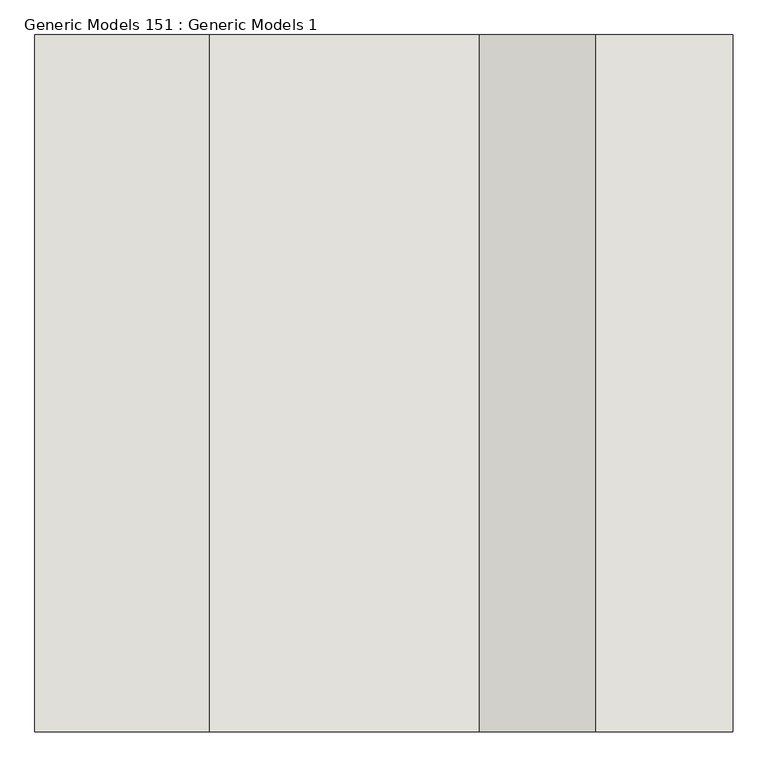
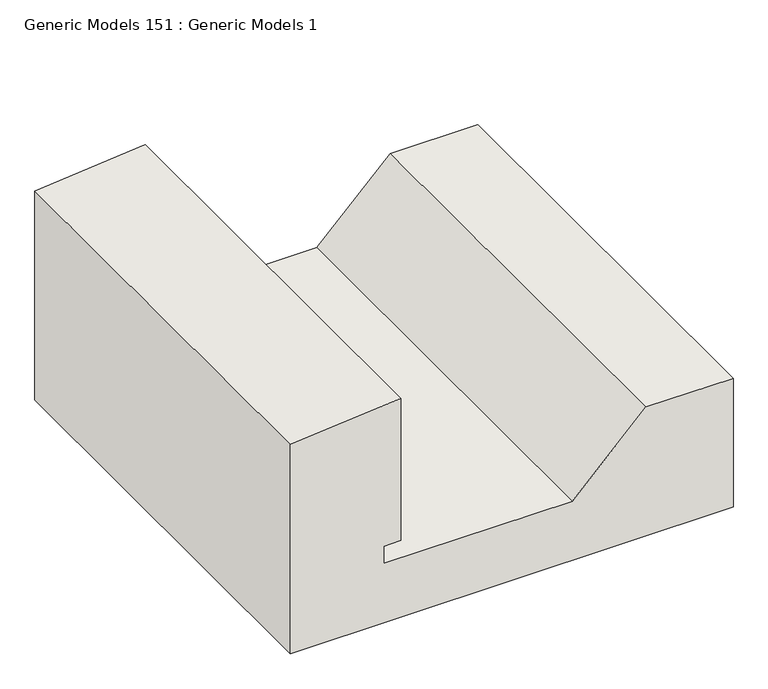
"""IFC4 building model written with IfcOpenShell, lengths in millimetres: wall geometry, Generic Models 151 : Generic Models 1."""

from ifc_helpers import new_model, si_unit, frame, origin, place, context, project, spatial, polyline, outline, extrude, source, transform, mapped, element, save


def generic_models_151_generic_models_1_08f1ca75(model_context):
    return source(origin(), model_context, "Body", "SweptSolid", [
        extrude(outline(polyline([(-76.2, 51566.7625), (-685.8, 51566.7625), (-685.8, 52787.3395874), (-310.1710164, 52787.3395874), (-310.1710164, 52546.8563593), (-513.3710164, 52343.6563593), (-513.3710164, 51824.8420742), (-462.5710164, 51824.8420742), (-462.5710164, 51871.5625), (-47.9216734, 51871.5625), (-76.2, 51566.7625)])), frame((0.0, 0.0, 0.0), z_axis=(0.0, 1.0, 0.0), x_axis=(0.0, 0.0, 1.0)), (0.0, 0.0, 1.0), 1219.2),
    ])


if __name__ == "__main__":
    model = new_model("IFC4")
    model_context = context("Model", 3, world=origin())
    ifc_project = project(units=[si_unit("LENGTHUNIT", "METRE", prefix="MILLI")], contexts=[model_context])
    site = spatial("IfcSite", under=ifc_project)
    building = spatial("IfcBuilding", under=site)
    placement = place(None, origin())
    generic_models_151_generic_models_1_shape = generic_models_151_generic_models_1_08f1ca75(model_context)
    element("IfcWall", 1, ObjectType="Generic Models 151 : Generic Models 1", at=placement, inside=building, context=model_context, shape_type="MappedRepresentation", body=[
        mapped(generic_models_151_generic_models_1_shape, transform((0.0, 0.0, 0.0), x_axis=(1.0, 0.0, 0.0), y_axis=(0.0, 1.0, 0.0), z_axis=(0.0, 0.0, 1.0))),
    ])
    save(model, "model.ifc")

# Revit data of these elements
# Element 1 (IfcWall, "Generic Models 151 : Generic Models 1")
#   Materials on its faces: "GRADE (SLOPE 2% MIN AWAY FROM BUILDING)"
# Materials
#   "GRADE (SLOPE 2% MIN AWAY FROM BUILDING)": class "Generic", colour RGB 211 211 211, transparency 0, Description = "Soil", Cost = 0
